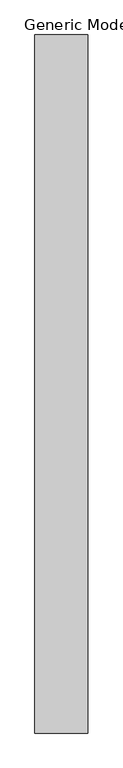
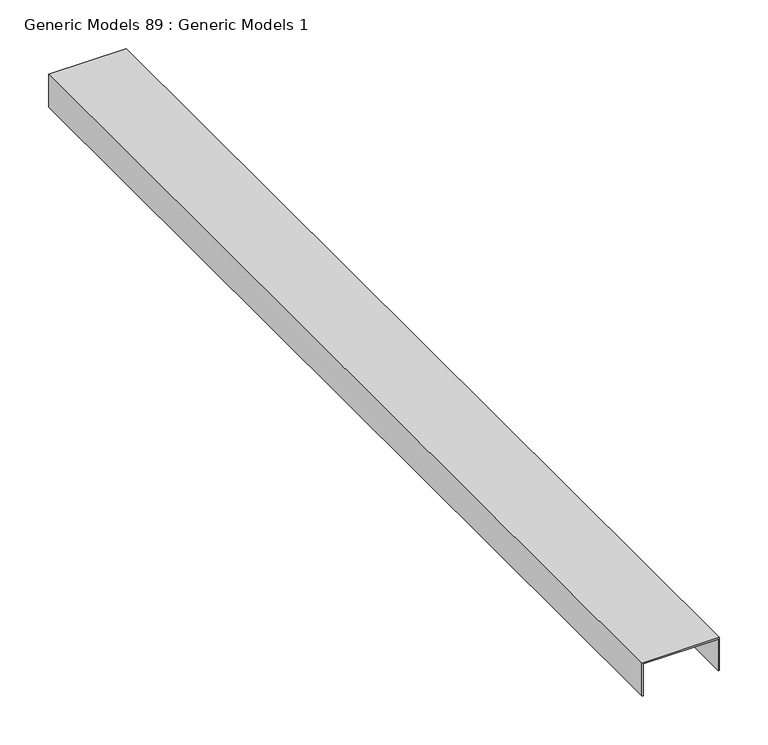
"""IFC4 building model written with IfcOpenShell, lengths in millimetres: proxy geometry, Generic Models 89 : Generic Models 1."""

from ifc_helpers import new_model, si_unit, frame, origin, place, context, project, spatial, polyline, outline, extrude, source, transform, mapped, element, save


def generic_models_89_generic_models_1_c4ef7a47(model_context):
    return source(origin(), model_context, "Body", "SweptSolid", [
        extrude(outline(polyline([(294.3266124, 48583.1181639), (294.3266124, 48491.0431639), (253.0516124, 48491.0431639), (253.0516124, 48492.6306639), (292.7391124, 48492.6306639), (292.7391124, 48581.5306639), (253.0516124, 48581.5306639), (253.0516124, 48583.1181639), (294.3266124, 48583.1181639)])), frame((0.0, 0.0, 0.0), z_axis=(0.0, 1.0, 0.0), x_axis=(0.0, 0.0, 1.0)), (0.0, 0.0, 1.0), 1219.2),
    ])


if __name__ == "__main__":
    model = new_model("IFC4")
    model_context = context("Model", 3, world=origin())
    ifc_project = project(units=[si_unit("LENGTHUNIT", "METRE", prefix="MILLI")], contexts=[model_context])
    site = spatial("IfcSite", under=ifc_project)
    building = spatial("IfcBuilding", under=site)
    placement = place(None, origin())
    generic_models_89_generic_models_1_shape = generic_models_89_generic_models_1_c4ef7a47(model_context)
    element("IfcBuildingElementProxy", 1, Name="Generic Models 89 : Generic Models 1", ObjectType="Generic Models 89 : Generic Models 1", at=placement, inside=building, context=model_context, shape_type="MappedRepresentation", body=[
        mapped(generic_models_89_generic_models_1_shape, transform((0.0, 0.0, 0.0), x_axis=(1.0, 0.0, 0.0), y_axis=(0.0, 1.0, 0.0), z_axis=(0.0, 0.0, 1.0))),
    ])
    save(model, "model.ifc")

# Revit data of these elements
# Element 1 (IfcBuildingElementProxy, "Generic Models 89 : Generic Models 1")
#   Materials on its faces: "METAL RUNNER CHANNEL TO RUN CONTINOUS FROM WALL TO WALL (ANCHOR AT BOTH ENDS)"
# Materials
#   "METAL RUNNER CHANNEL TO RUN CONTINOUS FROM WALL TO WALL (ANCHOR AT BOTH ENDS)": class "Unassigned", colour RGB 210 209 208, transparency 0, Keynote = "M05121300.02", Cost = 0
